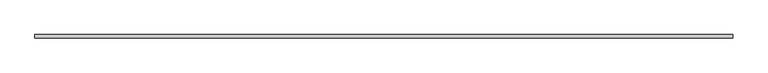
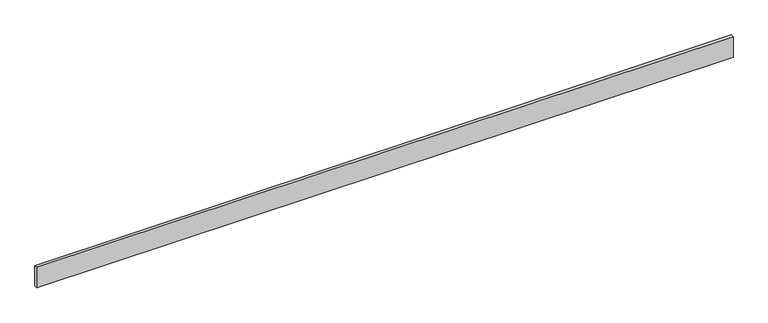
"""IFC4 building model written with IfcOpenShell, lengths in millimetres: proxy geometry, Generic Models 7:Generic Models 1:6:Generic Models 1:6 : Generic Models 7:Generic Models 1:337419:4 : Generic Models 7:Generic Models 1:6:Generic Models 1:6 : Generic Models 7:Generic Models 1:337419:312901."""

from ifc_helpers import new_model, si_unit, frame, origin, place, context, project, spatial, polyline, outline, extrude, source, transform, mapped, element, save


def generic_models_7aebc4ff(model_context):
    return source(origin(), model_context, "Body", "SweptSolid", [
        extrude(outline(polyline([(602310.5867239, -578937.1913841), (602310.5867239, -579140.3913841), (557809.7867239, -579140.3913841), (557809.7867239, -578937.1913841), (602310.5867239, -578937.1913841)])), frame((0.0, 0.0, -1377.3372439), z_axis=(0.0, 0.0, 1.0), x_axis=(1.0, 0.0, 0.0)), (0.0, 0.0, 1.0), 1377.3372439),
    ])


if __name__ == "__main__":
    model = new_model("IFC4")
    model_context = context("Model", 3, world=origin())
    ifc_project = project(units=[si_unit("LENGTHUNIT", "METRE", prefix="MILLI")], contexts=[model_context])
    site = spatial("IfcSite", under=ifc_project)
    building = spatial("IfcBuilding", under=site)
    placement = place(None, origin())
    generic_models_shape = generic_models_7aebc4ff(model_context)
    element("IfcBuildingElementProxy", 1, Name="Generic Models 7:Generic Models 1:6:Generic Models 1:6 : Generic Models 7:Generic Models 1:337419:4 : Generic Models 7:Generic Models 1:6:Generic Models 1:6 : Generic Models 7:Generic Models 1:337419:312901", ObjectType="Generic Models 7:Generic Models 1:6:Generic Models 1:6 : Generic Models 7:Generic Models 1:337419:4 : Generic Models 7:Generic Models 1:6:Generic Models 1:6 : Generic Models 7:Generic Models 1:337419:312901", at=placement, inside=building, context=model_context, shape_type="MappedRepresentation", body=[
        mapped(generic_models_shape, transform((0.0, 0.0, 0.0), x_axis=(1.0, 0.0, 0.0), y_axis=(0.0, 1.0, 0.0), z_axis=(0.0, 0.0, 1.0))),
    ])
    save(model, "model.ifc")

# Revit data of these elements
# Type "Generic Models 7:Generic Models 1:6:Generic Models 1:6 : Generic Models 7:Generic Models 1:337419:4 : Generic Models 7:Generic Models 1:6:Generic Models 1:6 : Generic Models 7:Generic Models 1:337419:312901"
#   NameOverride = "Generic Models 7:Generic Models 1:6:Generic Models 1:6 : Generic Models 7:Generic Models 1:337419:312901"
#   ObjectTypeOverride = "Generic Models 1:6 : Generic Models 7:Generic Models 1:337419"
#   Reference = "Generic Models 1"
#   Tag = "312901"
# Element 1 (IfcBuildingElementProxy, "Generic Models 7:Generic Models 1:6:Generic Models 1:6 : Generic Models 7:Generic Models 1:337419:4 : Generic Models 7:Generic Models 1:6:Generic Models 1:6 : Generic Models 7:Generic Models 1:337419:312901")
#   Materials on its faces: "CONCRETE FROST WALL - SEE STRUCT DWGS."
# Materials
#   "CONCRETE FROST WALL - SEE STRUCT DWGS.": class "Concrete", colour RGB 115 116 108, transparency 0, Description = "Lightweight concrete", Cost = 0
